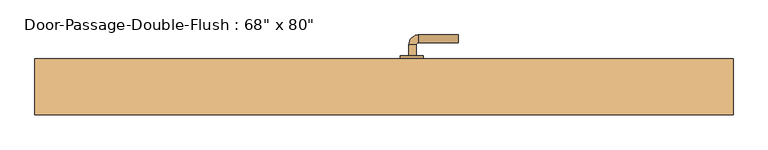
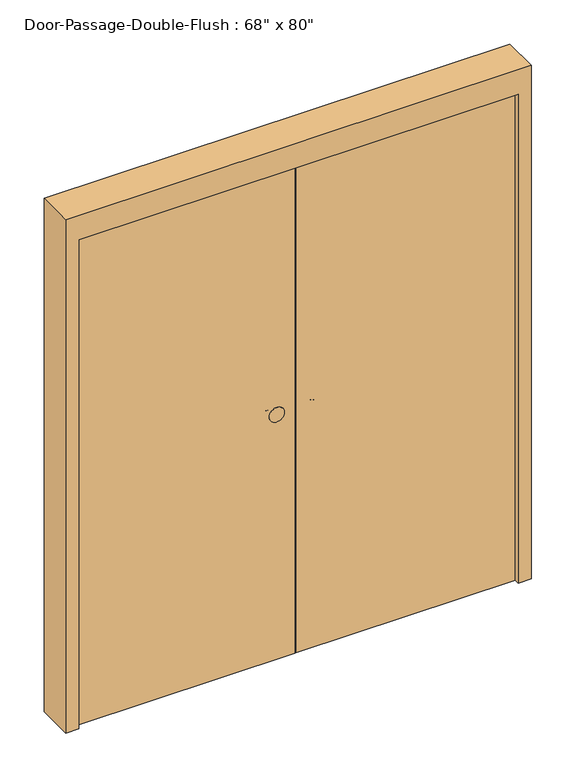
"""IFC4 building model written with IfcOpenShell, lengths in millimetres: door geometry."""

import ifcopenshell
import ifcopenshell.guid

model = None  # the IFC model being written
_history = None  # IfcOwnerHistory: only IFC2X3 demands one
_inside = {}  # id of a spatial element -> (the spatial element, [elements in it])
_under = {}  # id of a project, library or spatial element -> (it, [spatial elements below it])
_declared = {}  # id of a project -> (the project, [libraries it declares])
_typed = {}  # id of a type object -> (the type object, [elements of that type])
_made_of = {}  # id of a material, layer set ... -> (it, [elements and type objects made of it])


def new_model(schema):
    """Start an empty IFC model of exactly this schema.

    Asked for "IFC4X3", IfcOpenShell would pick the latest addendum, in which some entities
    have other attributes; the version numbers below select the first issue.
    IFC2X3 requires an IfcOwnerHistory on every rooted entity: one is made here for all.
    """
    global model, _history
    if schema == "IFC4X3":
        model = ifcopenshell.file(schema_version=(4, 3, 0, 0))
    else:
        model = ifcopenshell.file(schema=schema)
    _inside.clear()
    _under.clear()
    _declared.clear()
    _typed.clear()
    _made_of.clear()
    _history = None
    if model.schema == "IFC2X3":
        org = make("IfcOrganization", Name="unknown")
        user = make(
            "IfcPersonAndOrganization",
            ThePerson=make("IfcPerson", FamilyName="unknown"),
            TheOrganization=org,
        )
        app = make(
            "IfcApplication",
            ApplicationDeveloper=org,
            Version="unknown",
            ApplicationFullName="unknown",
            ApplicationIdentifier="unknown",
        )
        _history = make(
            "IfcOwnerHistory",
            OwningUser=user,
            OwningApplication=app,
            ChangeAction="ADDED",
            CreationDate=0,
        )
    return model


def make(cls, **values):
    """One entity of the class cls with the attributes given. An attribute that is None is left unset."""
    return model.create_entity(
        cls, **{name: value for name, value in values.items() if value is not None}
    )


def rooted(cls, **values):
    """An entity with a GlobalId (a new one), such as an element, a storey or a relation."""
    return make(cls, GlobalId=ifcopenshell.guid.new(), OwnerHistory=_history, **values)


def si_unit(unit_type, name, prefix=None):
    """IfcSIUnit, for example si_unit("LENGTHUNIT", "METRE", prefix="MILLI")."""
    return make("IfcSIUnit", UnitType=unit_type, Prefix=prefix, Name=name)


def assignment(units):
    """IfcUnitAssignment: the units of a project."""
    return None if units is None else make("IfcUnitAssignment", Units=units)


def point(xyz):
    """IfcCartesianPoint."""
    return None if xyz is None else make("IfcCartesianPoint", Coordinates=xyz)


def direction(xyz):
    """IfcDirection."""
    return None if xyz is None else make("IfcDirection", DirectionRatios=xyz)


def frame(location, z_axis=None, x_axis=None):
    """IfcAxis2Placement3D, a coordinate frame: its origin and axes. An axis left out is left unset."""
    return make(
        "IfcAxis2Placement3D",
        Location=point(location),
        Axis=direction(z_axis),
        RefDirection=direction(x_axis),
    )


def frame_2d(location, x_axis=None):
    """IfcAxis2Placement2D, a coordinate frame in the plane: its origin and x axis."""
    return make(
        "IfcAxis2Placement2D", Location=point(location), RefDirection=direction(x_axis)
    )


def origin():
    """The frame at (0, 0, 0) with its axes left unset."""
    return frame((0.0, 0.0, 0.0))


def origin_with_axes():
    """The frame at (0, 0, 0) with the z axis (0, 0, 1) and the x axis (1, 0, 0) written out."""
    return frame((0.0, 0.0, 0.0), z_axis=(0.0, 0.0, 1.0), x_axis=(1.0, 0.0, 0.0))


def place(relative_to, where):
    """IfcLocalPlacement: puts the frame where relative to a parent placement (None: the world)."""
    return make(
        "IfcLocalPlacement", PlacementRelTo=relative_to, RelativePlacement=where
    )


def context(
    kind, dimensions, precision=None, world=None, true_north=None, identifier=None
):
    """IfcGeometricRepresentationContext, for example the 3D "Model" context."""
    return make(
        "IfcGeometricRepresentationContext",
        ContextIdentifier=identifier,
        ContextType=kind,
        CoordinateSpaceDimension=dimensions,
        Precision=precision,
        WorldCoordinateSystem=world,
        TrueNorth=true_north,
    )


def project(units=None, contexts=None):
    """IfcProject with its units and contexts."""
    return rooted(
        "IfcProject",
        Name="project",
        RepresentationContexts=contexts,
        UnitsInContext=assignment(units),
    )


def spatial(cls, under=None, at=None, **own):
    """A site, building, storey or space (cls), placed at a placement, below another one or the project."""
    s = rooted(cls, ObjectPlacement=at, **own)
    if under is not None:
        _under.setdefault(under.id(), (under, []))[1].append(s)
    return s


def polyline(points):
    """IfcPolyline through the points."""
    return make("IfcPolyline", Points=[point(p) for p in points])


def circle_curve(where, radius):
    """IfcCircle in the frame where."""
    return make("IfcCircle", Position=where, Radius=radius)


def ellipse_curve(where, semi_axis1, semi_axis2):
    """IfcEllipse in the frame where."""
    return make(
        "IfcEllipse", Position=where, SemiAxis1=semi_axis1, SemiAxis2=semi_axis2
    )


def trimmed(basis, trim1, trim2, sense, master):
    """IfcTrimmedCurve: the piece of a basis curve between two trims."""
    return make(
        "IfcTrimmedCurve",
        BasisCurve=basis,
        Trim1=trim1,
        Trim2=trim2,
        SenseAgreement=sense,
        MasterRepresentation=master,
    )


def segment(curve, same_sense, transition):
    """IfcCompositeCurveSegment."""
    return make(
        "IfcCompositeCurveSegment",
        Transition=transition,
        SameSense=same_sense,
        ParentCurve=curve,
    )


def composite_curve(segments, self_intersect=None):
    """IfcCompositeCurve: segments joined end to end."""
    return make("IfcCompositeCurve", Segments=segments, SelfIntersect=self_intersect)


def outline(outer, holes=None, kind="AREA"):
    """IfcArbitraryClosedProfileDef: a profile drawn as a closed curve; with holes, ...WithVoids."""
    if holes is None:
        return make("IfcArbitraryClosedProfileDef", ProfileType=kind, OuterCurve=outer)
    return make(
        "IfcArbitraryProfileDefWithVoids",
        ProfileType=kind,
        OuterCurve=outer,
        InnerCurves=holes,
    )


def extrude(swept, where, along, depth):
    """IfcExtrudedAreaSolid: the profile swept, set in the frame where, extruded along a direction by depth."""
    return make(
        "IfcExtrudedAreaSolid",
        SweptArea=swept,
        Position=where,
        ExtrudedDirection=direction(along),
        Depth=depth,
    )


def faces_of(points, faces, orient=None, outer=None):
    """IfcFace entities. A face is a list of loops; a loop is a list of indices into points, from 0.

    orient and outer hold one flag for each loop. By default every Orientation is true, the
    first loop of a face is its IfcFaceOuterBound and the others are IfcFaceBound.
    """
    made = []
    for i, loops in enumerate(faces):
        bounds = []
        for j, loop in enumerate(loops):
            is_outer = j == 0 if outer is None else outer[i][j]
            bounds.append(
                make(
                    "IfcFaceOuterBound" if is_outer else "IfcFaceBound",
                    Bound=make("IfcPolyLoop", Polygon=[points[k] for k in loop]),
                    Orientation=True if orient is None else orient[i][j],
                )
            )
        made.append(make("IfcFace", Bounds=bounds))
    return made


def faceted_brep(points, faces, orient=None, outer=None, voids=None):
    """IfcFacetedBrep: a solid bounded by flat faces; with voids (closed shells), ...WithVoids."""
    shared = [point(p) for p in points]
    hull = make("IfcClosedShell", CfsFaces=faces_of(shared, faces, orient, outer))
    if voids is None:
        return make("IfcFacetedBrep", Outer=hull)
    return make(
        "IfcFacetedBrepWithVoids",
        Outer=hull,
        Voids=[
            make(cls, CfsFaces=faces_of(shared, fs, o, b)) for cls, fs, o, b in voids
        ],
    )


def shape(context_of_items, identifier, shape_type, items):
    """IfcShapeRepresentation: the items that make up one representation, for example the "Body"."""
    return make(
        "IfcShapeRepresentation",
        ContextOfItems=context_of_items,
        RepresentationIdentifier=identifier,
        RepresentationType=shape_type,
        Items=items,
    )


def source(mapping_origin, context_of_items, identifier, shape_type, items):
    """IfcRepresentationMap: a shape defined once, which mapped items show again and again."""
    return make(
        "IfcRepresentationMap",
        MappingOrigin=mapping_origin,
        MappedRepresentation=shape(context_of_items, identifier, shape_type, items),
    )


def transform(
    local_origin,
    x_axis=None,
    y_axis=None,
    z_axis=None,
    scale=None,
    scale2=None,
    scale3=None,
    uniform=True,
):
    """IfcCartesianTransformationOperator3D, or its non-uniform kind. x_axis, y_axis, z_axis: its Axis1, 2, 3."""
    if uniform:
        return make(
            "IfcCartesianTransformationOperator3D",
            Axis1=direction(x_axis),
            Axis2=direction(y_axis),
            LocalOrigin=point(local_origin),
            Scale=scale,
            Axis3=direction(z_axis),
        )
    return make(
        "IfcCartesianTransformationOperator3DnonUniform",
        Axis1=direction(x_axis),
        Axis2=direction(y_axis),
        LocalOrigin=point(local_origin),
        Scale=scale,
        Axis3=direction(z_axis),
        Scale2=scale2,
        Scale3=scale3,
    )


def mapped(mapping_source, mapping_target):
    """IfcMappedItem: shows the shape of a source again, moved by a transform."""
    return make(
        "IfcMappedItem", MappingSource=mapping_source, MappingTarget=mapping_target
    )


def made_of(thing, what):
    """Note that an element or type object is made of a material, layer set ...; save() writes the relation."""
    if what is not None:
        _made_of.setdefault(what.id(), (what, []))[1].append(thing)
    return thing


def element(
    cls,
    number,
    at=None,
    inside=None,
    cuts=None,
    type_object=None,
    material=None,
    context=None,
    identifier="Body",
    shape_type=None,
    held_by="IfcProductDefinitionShape",
    body=None,
    shapes=None,
    **own,
):
    """One element of the class cls, such as IfcWall. Its Tag is "e" and its number.

    at: its placement. inside: the storey or other place that contains it. cuts: it is an
    opening in that element (IfcRelVoidsElement). A single representation is given by context,
    identifier, shape_type and body (its items); several are given by shapes. held_by: the class
    of the entity that holds the representations. save() writes the other relations.
    """
    e = rooted(cls, Tag="e%d" % number, ObjectPlacement=at, **own)
    if body is not None:
        shapes = [shape(context, identifier, shape_type, body)]
    if shapes is not None:
        e.Representation = make(held_by, Representations=shapes)
    if inside is not None:
        _inside.setdefault(inside.id(), (inside, []))[1].append(e)
    if cuts is not None:
        rooted(
            "IfcRelVoidsElement", RelatingBuildingElement=cuts, RelatedOpeningElement=e
        )
    if type_object is not None:
        _typed.setdefault(type_object.id(), (type_object, []))[1].append(e)
    return made_of(e, material)


def aggregate(whole, parts):
    """IfcRelAggregates: a whole, such as a stair, and the parts it consists of."""
    return rooted("IfcRelAggregates", RelatingObject=whole, RelatedObjects=parts)


def save(model, path):
    """Write the relations noted so far, then the file.

    IfcRelAggregates (storeys below a building ...), IfcRelContainedInSpatialStructure (elements
    in a storey), IfcRelDefinesByType, IfcRelAssociatesMaterial and IfcRelDeclares: one each for
    every whole, place, type object, material and project.
    """
    for whole, parts in _under.values():
        aggregate(whole, parts)
    for where, things in _inside.values():
        rooted(
            "IfcRelContainedInSpatialStructure",
            RelatedElements=things,
            RelatingStructure=where,
        )
    for kind, things in _typed.values():
        rooted("IfcRelDefinesByType", RelatedObjects=things, RelatingType=kind)
    for what, things in _made_of.values():
        rooted("IfcRelAssociatesMaterial", RelatedObjects=things, RelatingMaterial=what)
    for by, libraries in _declared.values():
        rooted("IfcRelDeclares", RelatingContext=by, RelatedDefinitions=libraries)
    model.write(path)


def plane_surface(at):
    """IfcPlane: the flat surface through the origin of the frame at, square to its z axis."""
    return make("IfcPlane", Position=at)


def cylinder_surface(at, radius):
    """IfcCylindricalSurface: all points at the distance radius from the z axis of the frame at."""
    return make("IfcCylindricalSurface", Position=at, Radius=radius)


def revolved_surface(curve, axis_point, axis_direction):
    """IfcSurfaceOfRevolution: the curve turned about the line through axis_point along axis_direction."""
    return make(
        "IfcSurfaceOfRevolution",
        SweptCurve=make("IfcArbitraryOpenProfileDef", ProfileType="CURVE", Curve=curve),
        AxisPosition=make("IfcAxis1Placement", Location=point(axis_point), Axis=direction(axis_direction)),
    )


def advanced_brep(points, edges, surfaces, faces):
    """IfcAdvancedBrep: a solid bounded by faces that lie on surfaces and meet in shared edges.

    An edge is (start, end): straight between two places in points (the first is 0);
    or (start, end, curve); or (start, end, curve, False) where it runs against its curve.
    A face is (place in surfaces, loops), or (place, loops, False) where it looks against
    its surface's normal. A loop lists edges by number (the first is 1), with a minus sign
    where the edge is run from its end to its start. The first loop is the outer one.
    """
    corners = [point(p) for p in points]
    vertices = [make("IfcVertexPoint", VertexGeometry=c) for c in corners]
    made = []
    for start, end, *more in edges:
        made.append(
            make(
                "IfcEdgeCurve",
                EdgeStart=vertices[start],
                EdgeEnd=vertices[end],
                EdgeGeometry=more[0] if more else make("IfcPolyline", Points=[corners[start], corners[end]]),
                SameSense=more[1] if len(more) > 1 else True,
            )
        )
    hull = []
    for where, loops, *sense in faces:
        bounds = []
        for j, loop in enumerate(loops):
            ring = [make("IfcOrientedEdge", EdgeElement=made[abs(k) - 1], Orientation=k > 0) for k in loop]
            bounds.append(
                make(
                    "IfcFaceOuterBound" if j == 0 else "IfcFaceBound",
                    Bound=make("IfcEdgeLoop", EdgeList=ring),
                    Orientation=True,
                )
            )
        hull.append(make("IfcAdvancedFace", Bounds=bounds, FaceSurface=surfaces[where], SameSense=sense[0] if sense else True))
    return make("IfcAdvancedBrep", Outer=make("IfcClosedShell", CfsFaces=hull))


def door_efda3cbc(model_context):
    return source(origin(), model_context, "Body", "SolidModel", [
        advanced_brep(
        [(-65.009375, 155.5125, 1016.0), (-85.009375, 155.5125, 1016.0), (-65.009375, 125.5125, 1016.0), (-85.009375, 125.5125, 1016.0), (-90.009375, 120.5125, 1016.0), (-90.009375, 100.5125, 1016.0), (-195.009375, 100.5125, 1016.0), (-195.009375, 120.5125, 1016.0)],
        [
            (0, 1, circle_curve(frame((-75.009375, 155.5125, 1016.0), z_axis=(0.0, 1.0, 0.0), x_axis=(-1.0, 0.0, 0.0)), 10.0)),
            (1, 0, circle_curve(frame((-75.009375, 155.5125, 1016.0), z_axis=(0.0, 1.0, 0.0), x_axis=(-1.0, 0.0, 0.0)), 10.0)),
            (0, 2),
            (2, 3, circle_curve(frame((-75.009375, 125.5125, 1016.0), z_axis=(0.0, 1.0, 0.0), x_axis=(-1.0, 0.0, 0.0)), 10.0)),
            (3, 1),
            (3, 2, circle_curve(frame((-75.009375, 125.5125, 1016.0), z_axis=(0.0, 1.0, 0.0), x_axis=(-1.0, 0.0, 0.0)), 10.0)),
            (4, 3, circle_curve(frame((-90.009375, 125.5125, 1016.0), z_axis=(0.0, 0.0, 1.0), x_axis=(1.0, 0.0, 0.0)), 5.0)),
            (2, 5, circle_curve(frame((-90.009375, 125.5125, 1016.0), z_axis=(0.0, 0.0, -1.0), x_axis=(1.0, 0.0, 0.0)), 25.0)),
            (5, 4, circle_curve(frame((-90.009375, 110.5125, 1016.0), z_axis=(1.0, 0.0, 0.0), x_axis=(0.0, 1.0, 0.0)), 10.0)),
            (4, 5, circle_curve(frame((-90.009375, 110.5125, 1016.0), z_axis=(1.0, 0.0, 0.0), x_axis=(0.0, 1.0, 0.0)), 10.0)),
            (6, 7, circle_curve(frame((-195.009375, 110.5125, 1016.0), z_axis=(-1.0, 0.0, 0.0), x_axis=(0.0, 1.0, 0.0)), 10.0)),
            (7, 6, circle_curve(frame((-195.009375, 110.5125, 1016.0), z_axis=(-1.0, 0.0, 0.0), x_axis=(0.0, 1.0, 0.0)), 10.0)),
            (5, 6),
            (7, 4),
        ],
        [
            plane_surface(frame((-75.009375, 155.5125, 1016.0), z_axis=(0.0, 1.0, 0.0), x_axis=(0.0, 0.0, 1.0))),
            cylinder_surface(frame((-75.009375, 155.5125, 1016.0), z_axis=(0.0, 1.0, 0.0), x_axis=(-1.0, 0.0, 0.0)), 10.0),
            revolved_surface(trimmed(ellipse_curve(frame((-75.009375, 125.5125, 1016.0), z_axis=(0.0, 1.0, 0.0), x_axis=(-1.0, 0.0, 0.0)), 10.0, 10.0), [point((-65.009375, 125.5125, 1016.0))], [point((-85.009375, 125.5125, 1016.0))], True, "CARTESIAN"), (-90.009375, 125.5125, 1016.0), (0.0, 0.0, -1.0)),
            revolved_surface(trimmed(ellipse_curve(frame((-75.009375, 125.5125, 1016.0), z_axis=(0.0, 1.0, 0.0), x_axis=(-1.0, 0.0, 0.0)), 10.0, 10.0), [point((-85.009375, 125.5125, 1016.0))], [point((-65.009375, 125.5125, 1016.0))], True, "CARTESIAN"), (-90.009375, 125.5125, 1016.0), (0.0, 0.0, -1.0)),
            plane_surface(frame((-195.009375, 110.5125, 1016.0), z_axis=(-1.0, 0.0, 0.0), x_axis=(0.0, 0.0, 1.0))),
            cylinder_surface(frame((-90.009375, 110.5125, 1016.0), z_axis=(1.0, 0.0, 0.0), x_axis=(0.0, 1.0, 0.0)), 10.0),
        ],
        [
            (0, [[1, 2]]),
            (1, [[-1, 3, 4, 5]]),
            (1, [[-2, -5, 6, -3]]),
            (2, [[7, -4, 8, 9]]),
            (3, [[-8, -6, -7, 10]]),
            (4, [[11, 12]]),
            (5, [[-9, 13, -12, 14]]),
            (5, [[-10, -14, -11, -13]]),
        ],
    ),
        extrude(outline(composite_curve([segment(trimmed(circle_curve(frame_2d((1016.0, -72.509375)), 30.0), [point((1016.0, -42.509375))], [point((1016.0, -102.509375))], False, "CARTESIAN"), True, "CONTINUOUS"), segment(trimmed(circle_curve(frame_2d((1016.0, -72.509375)), 30.0), [point((1016.0, -102.509375))], [point((1016.0, -42.509375))], False, "CARTESIAN"), True, "CONTINUOUS")], self_intersect=False)), frame((0.0, 155.5125, 0.0), z_axis=(0.0, 1.0, 0.0), x_axis=(0.0, 0.0, 1.0)), (0.0, 0.0, 1.0), 8.0),
        advanced_brep(
        [(-65.009375, 90.55, 1016.0), (-85.009375, 90.55, 1016.0), (-85.009375, 120.55, 1016.0), (-65.009375, 120.55, 1016.0), (-90.009375, 125.55, 1016.0), (-90.009375, 145.55, 1016.0), (-195.009375, 145.55, 1016.0), (-195.009375, 125.55, 1016.0)],
        [
            (0, 1, circle_curve(frame((-75.009375, 90.55, 1016.0), z_axis=(0.0, -1.0, 0.0), x_axis=(-1.0, 0.0, 0.0)), 10.0)),
            (1, 0, circle_curve(frame((-75.009375, 90.55, 1016.0), z_axis=(0.0, -1.0, 0.0), x_axis=(-1.0, 0.0, 0.0)), 10.0)),
            (1, 2),
            (2, 3, circle_curve(frame((-75.009375, 120.55, 1016.0), z_axis=(0.0, -1.0, 0.0), x_axis=(-1.0, 0.0, 0.0)), 10.0)),
            (3, 0),
            (3, 2, circle_curve(frame((-75.009375, 120.55, 1016.0), z_axis=(0.0, -1.0, 0.0), x_axis=(-1.0, 0.0, 0.0)), 10.0)),
            (4, 5, circle_curve(frame((-90.009375, 135.55, 1016.0), z_axis=(1.0, 0.0, 0.0), x_axis=(0.0, -1.0, 0.0)), 10.0)),
            (5, 3, circle_curve(frame((-90.009375, 120.55, 1016.0), z_axis=(0.0, 0.0, -1.0), x_axis=(1.0, 0.0, 0.0)), 25.0)),
            (2, 4, circle_curve(frame((-90.009375, 120.55, 1016.0), z_axis=(0.0, 0.0, 1.0), x_axis=(1.0, 0.0, 0.0)), 5.0)),
            (5, 4, circle_curve(frame((-90.009375, 135.55, 1016.0), z_axis=(1.0, 0.0, 0.0), x_axis=(0.0, -1.0, 0.0)), 10.0)),
            (6, 7, circle_curve(frame((-195.009375, 135.55, 1016.0), z_axis=(-1.0, 0.0, 0.0), x_axis=(0.0, -1.0, 0.0)), 10.0)),
            (7, 6, circle_curve(frame((-195.009375, 135.55, 1016.0), z_axis=(-1.0, 0.0, 0.0), x_axis=(0.0, -1.0, 0.0)), 10.0)),
            (4, 7),
            (6, 5),
        ],
        [
            plane_surface(frame((-75.009375, 90.55, 1016.0), z_axis=(0.0, -1.0, 0.0), x_axis=(0.0, 0.0, 1.0))),
            cylinder_surface(frame((-75.009375, 90.55, 1016.0), z_axis=(0.0, -1.0, 0.0), x_axis=(-1.0, 0.0, 0.0)), 10.0),
            revolved_surface(trimmed(ellipse_curve(frame((-75.009375, 120.55, 1016.0), z_axis=(0.0, 1.0, 0.0), x_axis=(-1.0, 0.0, 0.0)), 10.0, 10.0), [point((-65.009375, 120.55, 1016.0))], [point((-85.009375, 120.55, 1016.0))], True, "CARTESIAN"), (-90.009375, 120.55, 1016.0), (0.0, 0.0, -1.0)),
            revolved_surface(trimmed(ellipse_curve(frame((-75.009375, 120.55, 1016.0), z_axis=(0.0, 1.0, 0.0), x_axis=(-1.0, 0.0, 0.0)), 10.0, 10.0), [point((-85.009375, 120.55, 1016.0))], [point((-65.009375, 120.55, 1016.0))], True, "CARTESIAN"), (-90.009375, 120.55, 1016.0), (0.0, 0.0, -1.0)),
            plane_surface(frame((-195.009375, 135.55, 1016.0), z_axis=(-1.0, 0.0, 0.0), x_axis=(0.0, 0.0, 1.0))),
            cylinder_surface(frame((-90.009375, 135.55, 1016.0), z_axis=(1.0, 0.0, 0.0), x_axis=(0.0, -1.0, 0.0)), 10.0),
        ],
        [
            (0, [[1, 2]]),
            (1, [[3, 4, 5, -2]]),
            (1, [[-5, 6, -3, -1]]),
            (2, [[7, 8, -4, 9]]),
            (3, [[10, -9, -6, -8]]),
            (4, [[11, 12]]),
            (5, [[13, -11, 14, -7]]),
            (5, [[-14, -12, -13, -10]]),
        ],
    ),
        extrude(outline(composite_curve([segment(trimmed(circle_curve(frame_2d((1016.0, -72.509375)), 30.0), [point((1016.0, -42.509375))], [point((1016.0, -102.509375))], False, "CARTESIAN"), True, "CONTINUOUS"), segment(trimmed(circle_curve(frame_2d((1016.0, -72.509375)), 30.0), [point((1016.0, -102.509375))], [point((1016.0, -42.509375))], False, "CARTESIAN"), True, "CONTINUOUS")], self_intersect=False)), frame((0.0, 82.55, 0.0), z_axis=(0.0, 1.0, 0.0), x_axis=(0.0, 0.0, 1.0)), (0.0, 0.0, 1.0), 8.0),
        advanced_brep(
        [(65.009375, 155.5125, 1016.0), (85.009375, 155.5125, 1016.0), (85.009375, 125.5125, 1016.0), (65.009375, 125.5125, 1016.0), (90.009375, 120.5125, 1016.0), (90.009375, 100.5125, 1016.0), (195.009375, 100.5125, 1016.0), (195.009375, 120.5125, 1016.0)],
        [
            (0, 1, circle_curve(frame((75.009375, 155.5125, 1016.0), z_axis=(0.0, 1.0, 0.0), x_axis=(1.0, 0.0, 0.0)), 10.0)),
            (1, 0, circle_curve(frame((75.009375, 155.5125, 1016.0), z_axis=(0.0, 1.0, 0.0), x_axis=(1.0, 0.0, 0.0)), 10.0)),
            (1, 2),
            (2, 3, circle_curve(frame((75.009375, 125.5125, 1016.0), z_axis=(0.0, 1.0, 0.0), x_axis=(1.0, 0.0, 0.0)), 10.0)),
            (3, 0),
            (3, 2, circle_curve(frame((75.009375, 125.5125, 1016.0), z_axis=(0.0, 1.0, 0.0), x_axis=(1.0, 0.0, 0.0)), 10.0)),
            (4, 5, circle_curve(frame((90.009375, 110.5125, 1016.0), z_axis=(-1.0, 0.0, 0.0), x_axis=(0.0, 1.0, 0.0)), 10.0)),
            (5, 3, circle_curve(frame((90.009375, 125.5125, 1016.0), z_axis=(0.0, 0.0, -1.0), x_axis=(-1.0, 0.0, 0.0)), 25.0)),
            (2, 4, circle_curve(frame((90.009375, 125.5125, 1016.0), z_axis=(0.0, 0.0, 1.0), x_axis=(-1.0, 0.0, 0.0)), 5.0)),
            (5, 4, circle_curve(frame((90.009375, 110.5125, 1016.0), z_axis=(-1.0, 0.0, 0.0), x_axis=(0.0, 1.0, 0.0)), 10.0)),
            (6, 7, circle_curve(frame((195.009375, 110.5125, 1016.0), z_axis=(1.0, 0.0, 0.0), x_axis=(0.0, 1.0, 0.0)), 10.0)),
            (7, 6, circle_curve(frame((195.009375, 110.5125, 1016.0), z_axis=(1.0, 0.0, 0.0), x_axis=(0.0, 1.0, 0.0)), 10.0)),
            (4, 7),
            (6, 5),
        ],
        [
            plane_surface(frame((75.009375, 155.5125, 1016.0), z_axis=(0.0, 1.0, 0.0), x_axis=(0.0, 0.0, 1.0))),
            cylinder_surface(frame((75.009375, 155.5125, 1016.0), z_axis=(0.0, 1.0, 0.0), x_axis=(1.0, 0.0, 0.0)), 10.0),
            revolved_surface(trimmed(ellipse_curve(frame((75.009375, 125.5125, 1016.0), z_axis=(0.0, -1.0, 0.0), x_axis=(1.0, 0.0, 0.0)), 10.0, 10.0), [point((65.009375, 125.5125, 1016.0))], [point((85.009375, 125.5125, 1016.0))], True, "CARTESIAN"), (90.009375, 125.5125, 1016.0), (0.0, 0.0, -1.0)),
            revolved_surface(trimmed(ellipse_curve(frame((75.009375, 125.5125, 1016.0), z_axis=(0.0, -1.0, 0.0), x_axis=(1.0, 0.0, 0.0)), 10.0, 10.0), [point((85.009375, 125.5125, 1016.0))], [point((65.009375, 125.5125, 1016.0))], True, "CARTESIAN"), (90.009375, 125.5125, 1016.0), (0.0, 0.0, -1.0)),
            plane_surface(frame((195.009375, 110.5125, 1016.0), z_axis=(1.0, 0.0, 0.0), x_axis=(0.0, 0.0, 1.0))),
            cylinder_surface(frame((90.009375, 110.5125, 1016.0), z_axis=(-1.0, 0.0, 0.0), x_axis=(0.0, 1.0, 0.0)), 10.0),
        ],
        [
            (0, [[1, 2]]),
            (1, [[3, 4, 5, -2]]),
            (1, [[-5, 6, -3, -1]]),
            (2, [[7, 8, -4, 9]]),
            (3, [[10, -9, -6, -8]]),
            (4, [[11, 12]]),
            (5, [[13, -11, 14, -7]]),
            (5, [[-14, -12, -13, -10]]),
        ],
    ),
        extrude(outline(composite_curve([segment(trimmed(circle_curve(frame_2d((1016.0, 72.509375)), 30.0), [point((1016.0, 42.509375))], [point((1016.0, 102.509375))], False, "CARTESIAN"), True, "CONTINUOUS"), segment(trimmed(circle_curve(frame_2d((1016.0, 72.509375)), 30.0), [point((1016.0, 102.509375))], [point((1016.0, 42.509375))], False, "CARTESIAN"), True, "CONTINUOUS")], self_intersect=False)), frame((0.0, 155.5125, 0.0), z_axis=(0.0, 1.0, 0.0), x_axis=(0.0, 0.0, 1.0)), (0.0, 0.0, 1.0), 8.0),
        advanced_brep(
        [(65.009375, 215.9625, 1016.0), (85.009375, 215.9625, 1016.0), (65.009375, 245.9625, 1016.0), (85.009375, 245.9625, 1016.0), (90.009375, 250.9625, 1016.0), (90.009375, 270.9625, 1016.0), (195.009375, 270.9625, 1016.0), (195.009375, 250.9625, 1016.0)],
        [
            (0, 1, circle_curve(frame((75.009375, 215.9625, 1016.0), z_axis=(0.0, -1.0, 0.0), x_axis=(1.0, 0.0, 0.0)), 10.0)),
            (1, 0, circle_curve(frame((75.009375, 215.9625, 1016.0), z_axis=(0.0, -1.0, 0.0), x_axis=(1.0, 0.0, 0.0)), 10.0)),
            (0, 2),
            (2, 3, circle_curve(frame((75.009375, 245.9625, 1016.0), z_axis=(0.0, -1.0, 0.0), x_axis=(1.0, 0.0, 0.0)), 10.0)),
            (3, 1),
            (3, 2, circle_curve(frame((75.009375, 245.9625, 1016.0), z_axis=(0.0, -1.0, 0.0), x_axis=(1.0, 0.0, 0.0)), 10.0)),
            (4, 3, circle_curve(frame((90.009375, 245.9625, 1016.0), z_axis=(0.0, 0.0, 1.0), x_axis=(-1.0, 0.0, 0.0)), 5.0)),
            (2, 5, circle_curve(frame((90.009375, 245.9625, 1016.0), z_axis=(0.0, 0.0, -1.0), x_axis=(-1.0, 0.0, 0.0)), 25.0)),
            (5, 4, circle_curve(frame((90.009375, 260.9625, 1016.0), z_axis=(-1.0, 0.0, 0.0), x_axis=(0.0, -1.0, 0.0)), 10.0)),
            (4, 5, circle_curve(frame((90.009375, 260.9625, 1016.0), z_axis=(-1.0, 0.0, 0.0), x_axis=(0.0, -1.0, 0.0)), 10.0)),
            (6, 7, circle_curve(frame((195.009375, 260.9625, 1016.0), z_axis=(1.0, 0.0, 0.0), x_axis=(0.0, -1.0, 0.0)), 10.0)),
            (7, 6, circle_curve(frame((195.009375, 260.9625, 1016.0), z_axis=(1.0, 0.0, 0.0), x_axis=(0.0, -1.0, 0.0)), 10.0)),
            (5, 6),
            (7, 4),
        ],
        [
            plane_surface(frame((75.009375, 215.9625, 1016.0), z_axis=(0.0, -1.0, 0.0), x_axis=(0.0, 0.0, 1.0))),
            cylinder_surface(frame((75.009375, 215.9625, 1016.0), z_axis=(0.0, -1.0, 0.0), x_axis=(1.0, 0.0, 0.0)), 10.0),
            revolved_surface(trimmed(ellipse_curve(frame((75.009375, 245.9625, 1016.0), z_axis=(0.0, -1.0, 0.0), x_axis=(1.0, 0.0, 0.0)), 10.0, 10.0), [point((65.009375, 245.9625, 1016.0))], [point((85.009375, 245.9625, 1016.0))], True, "CARTESIAN"), (90.009375, 245.9625, 1016.0), (0.0, 0.0, -1.0)),
            revolved_surface(trimmed(ellipse_curve(frame((75.009375, 245.9625, 1016.0), z_axis=(0.0, -1.0, 0.0), x_axis=(1.0, 0.0, 0.0)), 10.0, 10.0), [point((85.009375, 245.9625, 1016.0))], [point((65.009375, 245.9625, 1016.0))], True, "CARTESIAN"), (90.009375, 245.9625, 1016.0), (0.0, 0.0, -1.0)),
            plane_surface(frame((195.009375, 260.9625, 1016.0), z_axis=(1.0, 0.0, 0.0), x_axis=(0.0, 0.0, 1.0))),
            cylinder_surface(frame((90.009375, 260.9625, 1016.0), z_axis=(-1.0, 0.0, 0.0), x_axis=(0.0, -1.0, 0.0)), 10.0),
        ],
        [
            (0, [[1, 2]]),
            (1, [[-1, 3, 4, 5]]),
            (1, [[-2, -5, 6, -3]]),
            (2, [[7, -4, 8, 9]]),
            (3, [[-8, -6, -7, 10]]),
            (4, [[11, 12]]),
            (5, [[-9, 13, -12, 14]]),
            (5, [[-10, -14, -11, -13]]),
        ],
    ),
        extrude(outline(composite_curve([segment(trimmed(circle_curve(frame_2d((1016.0, 72.509375)), 30.0), [point((1016.0, 42.509375))], [point((1016.0, 102.509375))], False, "CARTESIAN"), True, "CONTINUOUS"), segment(trimmed(circle_curve(frame_2d((1016.0, 72.509375)), 30.0), [point((1016.0, 102.509375))], [point((1016.0, 42.509375))], False, "CARTESIAN"), True, "CONTINUOUS")], self_intersect=False)), frame((0.0, 207.9625, 0.0), z_axis=(0.0, 1.0, 0.0), x_axis=(0.0, 0.0, 1.0)), (0.0, 0.0, 1.0), 8.0),
        faceted_brep([(863.6, 158.75, 0.0), (863.6, 207.9625, 0.0), (914.4, 207.9625, 0.0), (914.4, 61.9125, 0.0), (863.6, 61.9125, 0.0), (863.6, 111.125, 0.0), (847.725, 111.125, 0.0), (847.725, 158.75, 0.0), (863.6, 158.75, 2032.0), (863.6, 207.9625, 2032.0), (-863.6, 207.9625, 2032.0), (-863.6, 207.9625, 0.0), (-914.4, 207.9625, 0.0), (-914.4, 207.9625, 2133.6), (914.4, 207.9625, 2133.6), (914.4, 61.9125, 2133.6), (-914.4, 61.9125, 2133.6), (-914.4, 61.9125, 0.0), (-863.6, 61.9125, 0.0), (-863.6, 61.9125, 2032.0), (863.6, 61.9125, 2032.0), (863.6, 111.125, 2032.0), (-863.6, 111.125, 2032.0), (-863.6, 111.125, 0.0), (-847.725, 111.125, 0.0), (-847.725, 111.125, 2016.125), (847.725, 111.125, 2016.125), (847.725, 158.75, 2016.125), (-847.725, 158.75, 2016.125), (-847.725, 158.75, 0.0), (-863.6, 158.75, 0.0), (-863.6, 158.75, 2032.0)], [[[0, 1, 2, 3, 4, 5, 6, 7]], [[1, 0, 8, 9]], [[2, 1, 9, 10, 11, 12, 13, 14]], [[3, 2, 14, 15]], [[4, 3, 15, 16, 17, 18, 19, 20]], [[5, 4, 20, 21]], [[6, 5, 21, 22, 23, 24, 25, 26]], [[7, 6, 26, 27]], [[0, 7, 27, 28, 29, 30, 31, 8]], [[9, 8, 31, 10]], [[20, 19, 22, 21]], [[26, 25, 28, 27]], [[12, 11, 30, 29, 24, 23, 18, 17]], [[11, 10, 31, 30]], [[13, 12, 17, 16]], [[19, 18, 23, 22]], [[25, 24, 29, 28]], [[15, 14, 13, 16]]]),
        extrude(outline(polyline([(863.6, 82.55), (1.5875, 82.55), (1.5875, 163.5125), (863.6, 163.5125), (863.6, 82.55)])), origin_with_axes(), (0.0, 0.0, 1.0), 2032.0),
        extrude(outline(polyline([(-1.5875, 82.55), (-863.6, 82.55), (-863.6, 163.5125), (-1.5875, 163.5125), (-1.5875, 82.55)])), origin_with_axes(), (0.0, 0.0, 1.0), 2032.0),
    ])


if __name__ == "__main__":
    model = new_model("IFC4")
    model_context = context("Model", 3, world=origin())
    ifc_project = project(units=[si_unit("LENGTHUNIT", "METRE", prefix="MILLI")], contexts=[model_context])
    site = spatial("IfcSite", under=ifc_project)
    building = spatial("IfcBuilding", under=site)
    placement = place(None, origin())
    door_shape = door_efda3cbc(model_context)
    element("IfcDoor", 1, ObjectType="Door-Passage-Double-Flush : 68\" x 80\"", at=placement, inside=building, context=model_context, shape_type="MappedRepresentation", body=[
        mapped(door_shape, transform((0.0, 0.0, 0.0), x_axis=(1.0, 0.0, 0.0), y_axis=(0.0, 1.0, 0.0), z_axis=(0.0, 0.0, 1.0))),
    ])
    save(model, "model.ifc")

# Revit data of these elements
# Type "Door-Passage-Double-Flush : 68\" x 80\""
#   Type Mark = "66"
#   Assembly Code = "B2030200"
#   Analytic Construction = "Metal"
#   Thickness = 0' - 1 3/4"
#   Thermal Resistance (R) = 1.5338 (h·ft²·°F)/BTU
#   Swing Angle [instance default] = 90.00°
#   Strike Height = 3' - 4"
#   SinglePanelWidth = 2' - 10"
#   Rough Width [instance default] = 6' - 0"
#   Rough Height [instance default] = 7' - 0"
#   MFOpeningHeight [instance default] = 0' - 4"
#   MFOpeningWidth [instance default] = 0' - 4"
#   Inset Calculate [instance default] = 0' - 4"
#   Masonry Inset [instance default] = 0' - 1"
#   Height = 6' - 8"
#   Width = 5' - 8"
#   Heat Transfer Coefficient (U) = 0.6520 BTU/(h·ft²·°F)
#   Masonry Frame Depth = 0' - 5 3/4"
#   Masonry Frame [instance default] = yes
#   Function = 1
#   Dry Wall Frame [instance default] = no
#   Panel Material = Metal Door - Brindle
#   Frame Material = Metal - Painted - Grey
#   Door Handle Material = Metal - Aluminium
#   Visual Light Transmittance = 0
#   Solar Heat Gain Coefficient = 0
#   Wall Closure = (empty or 0)
# Element 1 (IfcDoor, "Door-Passage-Double-Flush : 68\" x 80\"")
#   Materials on its faces: "Metal - Aluminium", "Metal - Painted - Grey", "Metal Door - Brindle"
# Materials
#   "Metal Door - Brindle": class "Paint", colour RGB 164 133 98, transparency 0
#   "Metal - Painted - Grey": class "Paint", colour RGB 104 104 104, transparency 0
#   "Metal - Aluminium": class "Metal", colour RGB 244 244 244, transparency 0
